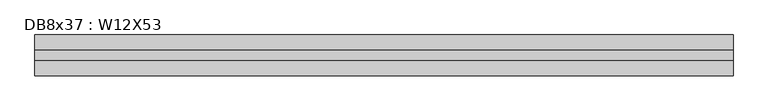
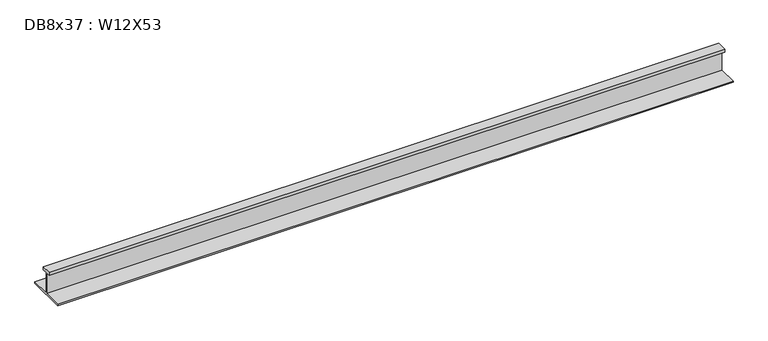
"""IFC4 building model written with IfcOpenShell, lengths in millimetres: beam geometry, DB8x37 : W12X53."""

from ifc_helpers import new_model, si_unit, frame, origin, place, context, project, spatial, polyline, outline, extrude, source, transform, mapped, element, save


def db8x37_w12x53_3b756228(model_context):
    return source(origin(), model_context, "Body", "SweptSolid", [
        extrude(outline(polyline([(38.1, 145.415), (38.1, 120.015), (2.921, 120.015), (2.921, -48.4505), (152.4, -48.4505), (152.4, -58.1025), (-152.4, -58.1025), (-152.4, -48.4505), (-2.921, -48.4505), (-2.921, 120.015), (-38.1, 120.015), (-38.1, 145.415), (38.1, 145.415)])), frame((-2606.929, 0.0, 0.0), z_axis=(1.0, 0.0, 0.0), x_axis=(0.0, 1.0, 0.0)), (0.0, 0.0, 1.0), 5213.858),
    ])


if __name__ == "__main__":
    model = new_model("IFC4")
    model_context = context("Model", 3, world=origin())
    ifc_project = project(units=[si_unit("LENGTHUNIT", "METRE", prefix="MILLI")], contexts=[model_context])
    site = spatial("IfcSite", under=ifc_project)
    building = spatial("IfcBuilding", under=site)
    placement = place(None, origin())
    db8x37_w12x53_shape = db8x37_w12x53_3b756228(model_context)
    element("IfcBeam", 1, ObjectType="DB8x37 : W12X53", at=placement, inside=building, context=model_context, shape_type="MappedRepresentation", body=[
        mapped(db8x37_w12x53_shape, transform((0.0, 0.0, 0.0), x_axis=(1.0, 0.0, 0.0), y_axis=(0.0, 1.0, 0.0), z_axis=(0.0, 0.0, 1.0))),
    ])
    save(model, "model.ifc")

# Revit data of these elements
# Type "DB8x37 : W12X53"
#   Assembly Code = "B10"
#   W = 53
#   Length [instance default] = 5' - 0"
#   bf = 0' - 10"
#   d = 1' - 0.1"
#   k = 0' - 1 3/8"
#   k2 = 0' - 0.8"
#   tf = 0' - 0.575"
#   tw = 0' - 0.345"
#   A = 0.108333 SF
#   Structural Material [instance default] = Steel ASTM A992
# Element 1 (IfcBeam, "DB8x37 : W12X53")
#   Materials on its faces: "Steel ASTM A992"
# Materials
#   "Steel ASTM A992": class "Metal", colour RGB 199 199 199, transparency 0, Description = "Structural steel 50ksi", Cost = 0
